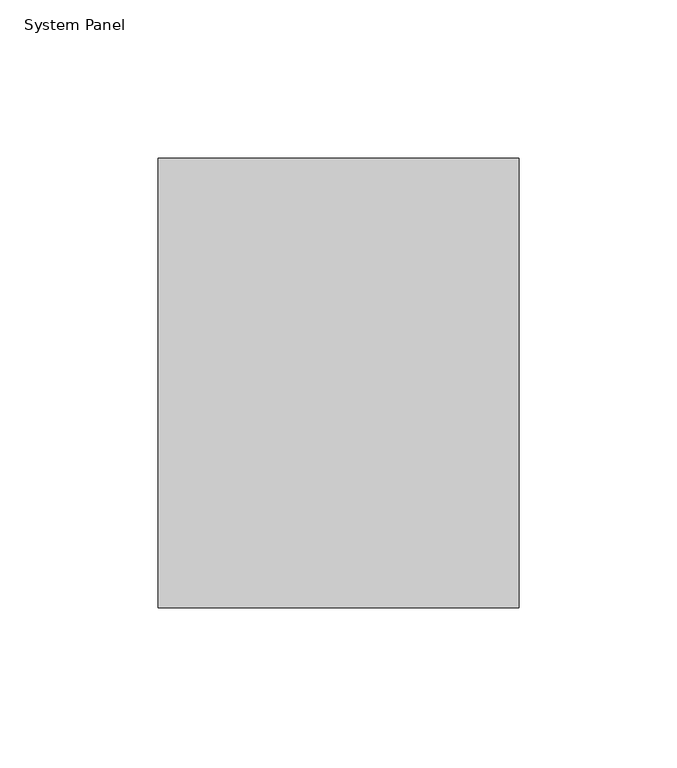
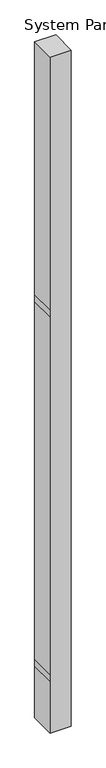
"""IFC4 building model written with IfcOpenShell, lengths in millimetres: plate geometry, System Panel : NLRS_21_CWP_hsb-vulling minerale wol 142 _gen_rsf."""

import ifcopenshell
import ifcopenshell.guid

model = None  # the IFC model being written
_history = None  # IfcOwnerHistory: only IFC2X3 demands one
_inside = {}  # id of a spatial element -> (the spatial element, [elements in it])
_under = {}  # id of a project, library or spatial element -> (it, [spatial elements below it])
_declared = {}  # id of a project -> (the project, [libraries it declares])
_typed = {}  # id of a type object -> (the type object, [elements of that type])
_made_of = {}  # id of a material, layer set ... -> (it, [elements and type objects made of it])


def new_model(schema):
    """Start an empty IFC model of exactly this schema.

    Asked for "IFC4X3", IfcOpenShell would pick the latest addendum, in which some entities
    have other attributes; the version numbers below select the first issue.
    IFC2X3 requires an IfcOwnerHistory on every rooted entity: one is made here for all.
    """
    global model, _history
    if schema == "IFC4X3":
        model = ifcopenshell.file(schema_version=(4, 3, 0, 0))
    else:
        model = ifcopenshell.file(schema=schema)
    _inside.clear()
    _under.clear()
    _declared.clear()
    _typed.clear()
    _made_of.clear()
    _history = None
    if model.schema == "IFC2X3":
        org = make("IfcOrganization", Name="unknown")
        user = make(
            "IfcPersonAndOrganization",
            ThePerson=make("IfcPerson", FamilyName="unknown"),
            TheOrganization=org,
        )
        app = make(
            "IfcApplication",
            ApplicationDeveloper=org,
            Version="unknown",
            ApplicationFullName="unknown",
            ApplicationIdentifier="unknown",
        )
        _history = make(
            "IfcOwnerHistory",
            OwningUser=user,
            OwningApplication=app,
            ChangeAction="ADDED",
            CreationDate=0,
        )
    return model


def make(cls, **values):
    """One entity of the class cls with the attributes given. An attribute that is None is left unset."""
    return model.create_entity(
        cls, **{name: value for name, value in values.items() if value is not None}
    )


def rooted(cls, **values):
    """An entity with a GlobalId (a new one), such as an element, a storey or a relation."""
    return make(cls, GlobalId=ifcopenshell.guid.new(), OwnerHistory=_history, **values)


def si_unit(unit_type, name, prefix=None):
    """IfcSIUnit, for example si_unit("LENGTHUNIT", "METRE", prefix="MILLI")."""
    return make("IfcSIUnit", UnitType=unit_type, Prefix=prefix, Name=name)


def assignment(units):
    """IfcUnitAssignment: the units of a project."""
    return None if units is None else make("IfcUnitAssignment", Units=units)


def point(xyz):
    """IfcCartesianPoint."""
    return None if xyz is None else make("IfcCartesianPoint", Coordinates=xyz)


def direction(xyz):
    """IfcDirection."""
    return None if xyz is None else make("IfcDirection", DirectionRatios=xyz)


def frame(location, z_axis=None, x_axis=None):
    """IfcAxis2Placement3D, a coordinate frame: its origin and axes. An axis left out is left unset."""
    return make(
        "IfcAxis2Placement3D",
        Location=point(location),
        Axis=direction(z_axis),
        RefDirection=direction(x_axis),
    )


def origin():
    """The frame at (0, 0, 0) with its axes left unset."""
    return frame((0.0, 0.0, 0.0))


def place(relative_to, where):
    """IfcLocalPlacement: puts the frame where relative to a parent placement (None: the world)."""
    return make(
        "IfcLocalPlacement", PlacementRelTo=relative_to, RelativePlacement=where
    )


def context(
    kind, dimensions, precision=None, world=None, true_north=None, identifier=None
):
    """IfcGeometricRepresentationContext, for example the 3D "Model" context."""
    return make(
        "IfcGeometricRepresentationContext",
        ContextIdentifier=identifier,
        ContextType=kind,
        CoordinateSpaceDimension=dimensions,
        Precision=precision,
        WorldCoordinateSystem=world,
        TrueNorth=true_north,
    )


def project(units=None, contexts=None):
    """IfcProject with its units and contexts."""
    return rooted(
        "IfcProject",
        Name="project",
        RepresentationContexts=contexts,
        UnitsInContext=assignment(units),
    )


def spatial(cls, under=None, at=None, **own):
    """A site, building, storey or space (cls), placed at a placement, below another one or the project."""
    s = rooted(cls, ObjectPlacement=at, **own)
    if under is not None:
        _under.setdefault(under.id(), (under, []))[1].append(s)
    return s


def polyline(points):
    """IfcPolyline through the points."""
    return make("IfcPolyline", Points=[point(p) for p in points])


def outline(outer, holes=None, kind="AREA"):
    """IfcArbitraryClosedProfileDef: a profile drawn as a closed curve; with holes, ...WithVoids."""
    if holes is None:
        return make("IfcArbitraryClosedProfileDef", ProfileType=kind, OuterCurve=outer)
    return make(
        "IfcArbitraryProfileDefWithVoids",
        ProfileType=kind,
        OuterCurve=outer,
        InnerCurves=holes,
    )


def extrude(swept, where, along, depth):
    """IfcExtrudedAreaSolid: the profile swept, set in the frame where, extruded along a direction by depth."""
    return make(
        "IfcExtrudedAreaSolid",
        SweptArea=swept,
        Position=where,
        ExtrudedDirection=direction(along),
        Depth=depth,
    )


def shape(context_of_items, identifier, shape_type, items):
    """IfcShapeRepresentation: the items that make up one representation, for example the "Body"."""
    return make(
        "IfcShapeRepresentation",
        ContextOfItems=context_of_items,
        RepresentationIdentifier=identifier,
        RepresentationType=shape_type,
        Items=items,
    )


def source(mapping_origin, context_of_items, identifier, shape_type, items):
    """IfcRepresentationMap: a shape defined once, which mapped items show again and again."""
    return make(
        "IfcRepresentationMap",
        MappingOrigin=mapping_origin,
        MappedRepresentation=shape(context_of_items, identifier, shape_type, items),
    )


def transform(
    local_origin,
    x_axis=None,
    y_axis=None,
    z_axis=None,
    scale=None,
    scale2=None,
    scale3=None,
    uniform=True,
):
    """IfcCartesianTransformationOperator3D, or its non-uniform kind. x_axis, y_axis, z_axis: its Axis1, 2, 3."""
    if uniform:
        return make(
            "IfcCartesianTransformationOperator3D",
            Axis1=direction(x_axis),
            Axis2=direction(y_axis),
            LocalOrigin=point(local_origin),
            Scale=scale,
            Axis3=direction(z_axis),
        )
    return make(
        "IfcCartesianTransformationOperator3DnonUniform",
        Axis1=direction(x_axis),
        Axis2=direction(y_axis),
        LocalOrigin=point(local_origin),
        Scale=scale,
        Axis3=direction(z_axis),
        Scale2=scale2,
        Scale3=scale3,
    )


def mapped(mapping_source, mapping_target):
    """IfcMappedItem: shows the shape of a source again, moved by a transform."""
    return make(
        "IfcMappedItem", MappingSource=mapping_source, MappingTarget=mapping_target
    )


def made_of(thing, what):
    """Note that an element or type object is made of a material, layer set ...; save() writes the relation."""
    if what is not None:
        _made_of.setdefault(what.id(), (what, []))[1].append(thing)
    return thing


def element(
    cls,
    number,
    at=None,
    inside=None,
    cuts=None,
    type_object=None,
    material=None,
    context=None,
    identifier="Body",
    shape_type=None,
    held_by="IfcProductDefinitionShape",
    body=None,
    shapes=None,
    **own,
):
    """One element of the class cls, such as IfcWall. Its Tag is "e" and its number.

    at: its placement. inside: the storey or other place that contains it. cuts: it is an
    opening in that element (IfcRelVoidsElement). A single representation is given by context,
    identifier, shape_type and body (its items); several are given by shapes. held_by: the class
    of the entity that holds the representations. save() writes the other relations.
    """
    e = rooted(cls, Tag="e%d" % number, ObjectPlacement=at, **own)
    if body is not None:
        shapes = [shape(context, identifier, shape_type, body)]
    if shapes is not None:
        e.Representation = make(held_by, Representations=shapes)
    if inside is not None:
        _inside.setdefault(inside.id(), (inside, []))[1].append(e)
    if cuts is not None:
        rooted(
            "IfcRelVoidsElement", RelatingBuildingElement=cuts, RelatedOpeningElement=e
        )
    if type_object is not None:
        _typed.setdefault(type_object.id(), (type_object, []))[1].append(e)
    return made_of(e, material)


def aggregate(whole, parts):
    """IfcRelAggregates: a whole, such as a stair, and the parts it consists of."""
    return rooted("IfcRelAggregates", RelatingObject=whole, RelatedObjects=parts)


def save(model, path):
    """Write the relations noted so far, then the file.

    IfcRelAggregates (storeys below a building ...), IfcRelContainedInSpatialStructure (elements
    in a storey), IfcRelDefinesByType, IfcRelAssociatesMaterial and IfcRelDeclares: one each for
    every whole, place, type object, material and project.
    """
    for whole, parts in _under.values():
        aggregate(whole, parts)
    for where, things in _inside.values():
        rooted(
            "IfcRelContainedInSpatialStructure",
            RelatedElements=things,
            RelatingStructure=where,
        )
    for kind, things in _typed.values():
        rooted("IfcRelDefinesByType", RelatedObjects=things, RelatingType=kind)
    for what, things in _made_of.values():
        rooted("IfcRelAssociatesMaterial", RelatedObjects=things, RelatingMaterial=what)
    for by, libraries in _declared.values():
        rooted("IfcRelDeclares", RelatingContext=by, RelatedDefinitions=libraries)
    model.write(path)


def system_panel_2185679e(model_context):
    return source(origin(), model_context, "Body", "SweptSolid", [
        extrude(outline(polyline([(0.0, -56.9999998), (0.0, 56.9999998), (295.0, 56.9999998), (333.0, 56.9999998), (2371.0, 56.9999998), (2409.0, 56.9999998), (3849.0, 56.9999998), (3849.0, -56.9999998), (2409.0, -56.9999998), (2371.0, -56.9999998), (333.0, -56.9999998), (295.0, -56.9999998), (0.0, -56.9999998)])), frame((0.0, -71.0, 0.0), z_axis=(0.0, 1.0, 0.0), x_axis=(0.0, 0.0, 1.0)), (0.0, 0.0, 1.0), 142.0),
    ])


if __name__ == "__main__":
    model = new_model("IFC4")
    model_context = context("Model", 3, world=origin())
    ifc_project = project(units=[si_unit("LENGTHUNIT", "METRE", prefix="MILLI")], contexts=[model_context])
    site = spatial("IfcSite", under=ifc_project)
    building = spatial("IfcBuilding", under=site)
    placement = place(None, origin())
    system_panel_shape = system_panel_2185679e(model_context)
    element("IfcPlate", 1, ObjectType="System Panel : NLRS_21_CWP_hsb-vulling minerale wol 142 _gen_rsf", at=placement, inside=building, context=model_context, shape_type="MappedRepresentation", body=[
        mapped(system_panel_shape, transform((0.0, 0.0, 0.0), x_axis=(1.0, 0.0, 0.0), y_axis=(0.0, 1.0, 0.0), z_axis=(0.0, 0.0, 1.0))),
    ])
    save(model, "model.ifc")

# Revit data of these elements
# Type "System Panel : NLRS_21_CWP_hsb-vulling minerale wol 142 _gen_rsf"
#   Export Type to IFC As = "IfcWall"
#   Type IfcGUID = "07M7mRoiH1CR8m_RSKIwpC"
#   Assembly Code = "21.23"
# Element 1 (IfcPlate, "System Panel : NLRS_21_CWP_hsb-vulling minerale wol 142 _gen_rsf")
#   Materials on its faces: "NLRS_m1_isolatie minerale wol_gen_rsf"
# Materials
#   "NLRS_m1_isolatie minerale wol_gen_rsf": class "M - Anorganische materialen", colour RGB 200 200 140, transparency 0, Keynote = "m1", Manufacturer = "Revit Standards Foundation", URL = "www.revitstandards.org", Description = "isolatie minerale wol", Cost = 0
